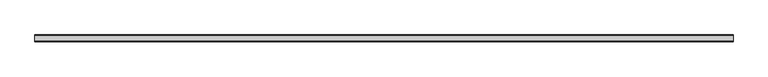
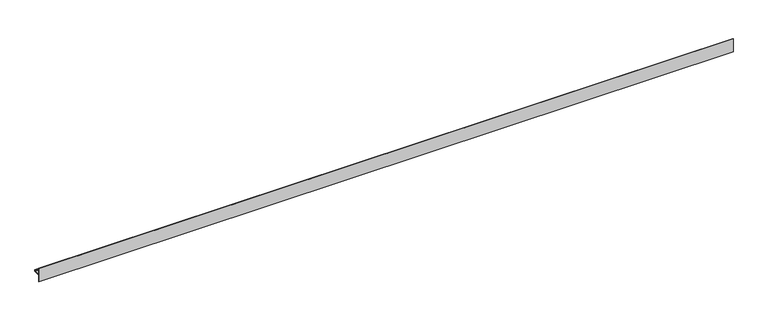
"""IFC4 building model written with IfcOpenShell, lengths in millimetres: proxy geometry, Metal profile008 3024 : Metal profile008 3024."""

from ifc_helpers import new_model, si_unit, frame, origin, place, context, project, spatial, polyline, outline, extrude, source, transform, mapped, element, save


def generic_models_cfdcdfcd(model_context):
    return source(origin(), model_context, "Body", "SweptSolid", [
        extrude(outline(polyline([(10465.7262552, 42924.8794763), (10465.7262552, 42920.1296763), (10447.4923073, 42920.1296763), (10447.4923073, 42901.0796763), (10446.2223073, 42901.0796763), (10446.2223073, 42940.4496763), (10447.4923073, 42940.4496763), (10447.4923073, 42921.3996763), (10464.4562552, 42921.3996763), (10464.4562552, 42924.8794763), (10465.7262552, 42924.8794763)])), frame((3694.2883192, 0.0, 0.0), z_axis=(1.0, 0.0, 0.0), x_axis=(0.0, 1.0, 0.0)), (0.0, 0.0, 1.0), 2000.0),
    ])


if __name__ == "__main__":
    model = new_model("IFC4")
    model_context = context("Model", 3, world=origin())
    ifc_project = project(units=[si_unit("LENGTHUNIT", "METRE", prefix="MILLI")], contexts=[model_context])
    site = spatial("IfcSite", under=ifc_project)
    building = spatial("IfcBuilding", under=site)
    placement = place(None, origin())
    generic_models_shape = generic_models_cfdcdfcd(model_context)
    element("IfcBuildingElementProxy", 1, Name="Metal profile008 3024 : Metal profile008 3024", ObjectType="Metal profile008 3024 : Metal profile008 3024", at=placement, inside=building, context=model_context, shape_type="MappedRepresentation", body=[
        mapped(generic_models_shape, transform((0.0, 0.0, 0.0), x_axis=(1.0, 0.0, 0.0), y_axis=(0.0, 1.0, 0.0), z_axis=(0.0, 0.0, 1.0))),
    ])
    save(model, "model.ifc")

# Revit data of these elements
# Type "Metal profile008 3024 : Metal profile008 3024"
#   NameOverride = "Metal profile008"
# Element 1 (IfcBuildingElementProxy, "Metal profile008 3024 : Metal profile008 3024")
#   Materials on its faces: "16 GA. COPPER VENTED T REVEAL BEAD"
# Materials
#   "16 GA. COPPER VENTED T REVEAL BEAD": class "Unassigned", colour RGB 255 227 10, transparency 0
